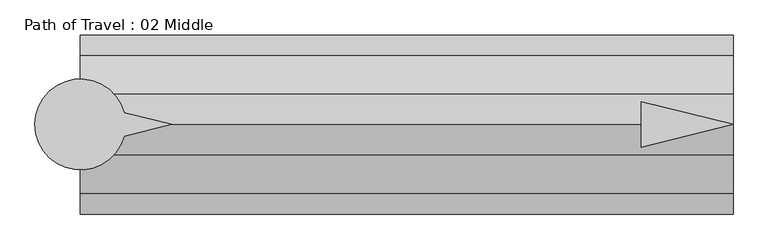
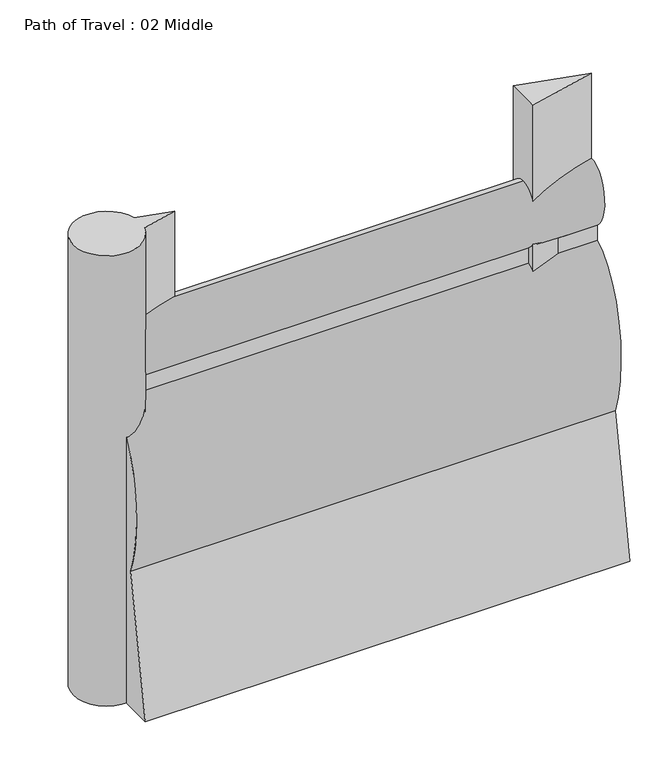
"""IFC4 building model written with IfcOpenShell, lengths in millimetres: proxy geometry, Path of Travel : 02 Middle."""

from ifc_helpers import new_model, si_unit, point, frame, frame_2d, origin, origin_with_axes, place, context, project, spatial, polyline, circle_curve, ellipse_curve, trimmed, segment, composite_curve, outline, extrude, source, transform, mapped, element, save
from ifc_brep_helpers import plane_surface, extruded_surface, advanced_brep


def path_of_travel_02_middle_73e1806b(model_context):
    return source(origin(), model_context, "Body", "SolidModel", [
        advanced_brep(
        [(227.5554837, 0.0, 1727.2), (227.5554837, 42.9018657, 1436.6534209), (227.5554837, 42.9018657, 1363.4763406), (227.5554837, 184.1186263, 643.4144547), (227.5554837, 297.5699544, 0.0), (227.5554837, 145.6574193, 0.0), (227.5554837, 0.0, 584.2), (227.5554837, -145.6574193, 0.0), (227.5554837, -297.5699544, 0.0), (227.5554837, -184.1186263, 643.4144547), (227.5554837, -42.9018657, 1363.4763406), (227.5554837, -42.9018657, 1436.6534209), (2397.3704554, 0.0, 1727.2), (2397.3704554, -42.9018657, 1436.6534209), (2397.3704554, -42.9018657, 1363.4763406), (2397.3704554, -184.1186263, 643.4144547), (2397.3704554, -297.5699544, 0.0), (2397.3704554, -145.6574193, 0.0), (2397.3704554, 0.0, 584.2), (2397.3704554, 145.6574193, 0.0), (2397.3704554, 297.5699544, 0.0), (2397.3704554, 184.1186263, 643.4144547), (2397.3704554, 42.9018657, 1363.4763406), (2397.3704554, 42.9018657, 1436.6534209)],
        [
            (0, 1, ellipse_curve(frame((227.5554837, 0.0, 1574.8), z_axis=(-1.0, 0.0, 0.0), x_axis=(0.0, 0.0, 1.0)), 152.4, 101.6)),
            (1, 2),
            (2, 3, ellipse_curve(frame((227.5554837, 0.0, 914.4), z_axis=(-1.0, 0.0, 0.0), x_axis=(0.0, 0.0, -1.0)), 457.2, 228.6)),
            (3, 4),
            (4, 5),
            (5, 6),
            (6, 7),
            (7, 8),
            (8, 9),
            (9, 10, ellipse_curve(frame((227.5554837, 0.0, 914.4), z_axis=(-1.0, 0.0, 0.0), x_axis=(0.0, 0.0, -1.0)), 457.2, 228.6)),
            (10, 11),
            (11, 0, ellipse_curve(frame((227.5554837, 0.0, 1574.8), z_axis=(-1.0, 0.0, 0.0), x_axis=(0.0, 0.0, 1.0)), 152.4, 101.6)),
            (12, 13, ellipse_curve(frame((2397.3704554, 0.0, 1574.8), z_axis=(1.0, 0.0, 0.0), x_axis=(0.0, 0.0, 1.0)), 152.4, 101.6)),
            (13, 14),
            (14, 15, ellipse_curve(frame((2397.3704554, 0.0, 914.4), z_axis=(1.0, 0.0, 0.0), x_axis=(0.0, 0.0, -1.0)), 457.2, 228.6)),
            (15, 16),
            (16, 17),
            (17, 18),
            (18, 19),
            (19, 20),
            (20, 21),
            (21, 22, ellipse_curve(frame((2397.3704554, 0.0, 914.4), z_axis=(1.0, 0.0, 0.0), x_axis=(0.0, 0.0, -1.0)), 457.2, 228.6)),
            (22, 23),
            (23, 12, ellipse_curve(frame((2397.3704554, 0.0, 1574.8), z_axis=(1.0, 0.0, 0.0), x_axis=(0.0, 0.0, 1.0)), 152.4, 101.6)),
            (0, 12),
            (23, 1),
            (22, 2),
            (21, 3),
            (20, 4),
            (19, 5),
            (18, 6),
            (17, 7),
            (16, 8),
            (15, 9),
            (14, 10),
            (13, 11),
        ],
        [
            plane_surface(frame((227.5554837, 0.0, 0.0), z_axis=(-1.0, 0.0, 0.0), x_axis=(0.0, 0.0, 1.0))),
            plane_surface(frame((2397.3704554, 0.0, 0.0), z_axis=(1.0, 0.0, 0.0), x_axis=(0.0, 0.0, 1.0))),
            extruded_surface(trimmed(ellipse_curve(frame((2397.3704554, 0.0, 1574.8), z_axis=(-1.0, 0.0, 0.0), x_axis=(0.0, 0.0, 1.0)), 152.4, 101.6), [point((2397.3704554, 0.0, 1727.2))], [point((2397.3704554, 42.9018657, 1436.6534209))], True, "CARTESIAN"), (-2169.8149717, 0.0, 0.0), 2169.8149717),
            plane_surface(frame((227.5554837, 42.9018657, 1436.6534209), z_axis=(0.0, 1.0, 0.0), x_axis=(1.0, 0.0, 0.0))),
            extruded_surface(trimmed(ellipse_curve(frame((2397.3704554, 0.0, 914.4), z_axis=(-1.0, 0.0, 0.0), x_axis=(0.0, 0.0, -1.0)), 457.2, 228.6), [point((2397.3704554, 42.9018657, 1363.4763406))], [point((2397.3704554, 184.1186263, 643.4144547))], True, "CARTESIAN"), (-2169.8149717, 0.0, 0.0), 2169.8149717),
            plane_surface(frame((227.5554837, 184.1186263, 643.4144547), z_axis=(0.0, 0.9848077530122078, 0.1736481776669322), x_axis=(1.0, 0.0, 0.0))),
            plane_surface(frame((227.5554837, 297.5699544, 0.0), z_axis=(0.0, 0.0, -1.0), x_axis=(1.0, 0.0, 0.0))),
            plane_surface(frame((227.5554837, 145.6574193, 0.0), z_axis=(0.0, -0.9702957262760199, -0.2419218955995739), x_axis=(1.0, 0.0, 0.0))),
            plane_surface(frame((227.5554837, 0.0, 584.2), z_axis=(0.0, 0.9702957262759961, -0.24192189559966923), x_axis=(1.0, 0.0, 0.0))),
            plane_surface(frame((227.5554837, -145.6574193, 0.0), z_axis=(0.0, 0.0, -1.0), x_axis=(1.0, 0.0, 0.0))),
            plane_surface(frame((227.5554837, -297.5699544, 0.0), z_axis=(0.0, -0.984807753012208, 0.17364817766693066), x_axis=(1.0, 0.0, 0.0))),
            extruded_surface(trimmed(ellipse_curve(frame((2397.3704554, 0.0, 914.4), z_axis=(-1.0, 0.0, 0.0), x_axis=(0.0, 0.0, -1.0)), 457.2, 228.6), [point((2397.3704554, -184.1186263, 643.4144547))], [point((2397.3704554, -42.9018657, 1363.4763406))], True, "CARTESIAN"), (-2169.8149717, 0.0, 0.0), 2169.8149717),
            plane_surface(frame((227.5554837, -42.9018657, 1363.4763406), z_axis=(0.0, -1.0, 0.0), x_axis=(1.0, 0.0, 0.0))),
            extruded_surface(trimmed(ellipse_curve(frame((2397.3704554, 0.0, 1574.8), z_axis=(-1.0, 0.0, 0.0), x_axis=(0.0, 0.0, 1.0)), 152.4, 101.6), [point((2397.3704554, -42.9018657, 1436.6534209))], [point((2397.3704554, 0.0, 1727.2))], True, "CARTESIAN"), (-2169.8149717, 0.0, 0.0), 2169.8149717),
        ],
        [
            (0, [[1, 2, 3, 4, 5, 6, 7, 8, 9, 10, 11, 12]]),
            (1, [[13, 14, 15, 16, 17, 18, 19, 20, 21, 22, 23, 24]]),
            (2, [[-1, 25, -24, 26]]),
            (3, [[-2, -26, -23, 27]]),
            (4, [[-3, -27, -22, 28]]),
            (5, [[-4, -28, -21, 29]]),
            (6, [[-5, -29, -20, 30]]),
            (7, [[-6, -30, -19, 31]]),
            (8, [[-7, -31, -18, 32]]),
            (9, [[-8, -32, -17, 33]]),
            (10, [[-9, -33, -16, 34]]),
            (11, [[-10, -34, -15, 35]]),
            (12, [[-11, -35, -14, 36]]),
            (13, [[-12, -36, -13, -25]]),
        ],
    ),
        extrude(outline(polyline([(2091.3653088, 76.2006338), (2397.3704554, 0.0), (2091.3653088, -76.2006338), (2091.3653088, 76.2006338)])), origin_with_axes(), (0.0, 0.0, 1.0), 2129.5973753),
        extrude(outline(composite_curve([segment(polyline([(372.7837828, 39.4440225), (531.182385, 0.0), (372.7837828, -39.4440225)]), True, "CONTINUOUS"), segment(trimmed(circle_curve(frame_2d((227.2200886, 0.0)), 150.8131956), [point((372.7837828, -39.4440225))], [point((372.7837828, 39.4440225))], False, "CARTESIAN"), True, "CONTINUOUS")], self_intersect=False)), origin_with_axes(), (0.0, 0.0, 1.0), 2129.5973753),
    ])


if __name__ == "__main__":
    model = new_model("IFC4")
    model_context = context("Model", 3, world=origin())
    ifc_project = project(units=[si_unit("LENGTHUNIT", "METRE", prefix="MILLI")], contexts=[model_context])
    site = spatial("IfcSite", under=ifc_project)
    building = spatial("IfcBuilding", under=site)
    placement = place(None, origin())
    path_of_travel_02_middle_shape = path_of_travel_02_middle_73e1806b(model_context)
    element("IfcBuildingElementProxy", 1, Name="Path of Travel : 02 Middle", ObjectType="Path of Travel : 02 Middle", at=placement, inside=building, context=model_context, shape_type="MappedRepresentation", body=[
        mapped(path_of_travel_02_middle_shape, transform((0.0, 0.0, 0.0), x_axis=(1.0, 0.0, 0.0), y_axis=(0.0, 1.0, 0.0), z_axis=(0.0, 0.0, 1.0))),
    ])
    save(model, "model.ifc")

# Revit data of these elements
# Type "Path of Travel : 02 Middle"
#   Path of Egress [instance default] = 4' - 0"
#   built-in parameter 1001306 [instance default] = 4 (stored number, unit not read)
#   Dot at Start = no
#   Arrow in Middle = yes
#   Arrow at End = no
#   Egress Path = none
# Element 1 (IfcBuildingElementProxy, "Path of Travel : 02 Middle")
#   Path of Egress = 7' - 1 109/256"
#   built-in parameter 1001306 = 7.11882 (stored number, unit not read)
#   Materials on its faces: "Egress Path Solid", "solid"
# Materials
#   "Egress Path Solid": class "Unassigned", colour RGB 255 128 64, transparency 0.75, Comments = "Rendering appearance not upgraded "
#   "solid": class "Generic", colour RGB 120 120 120, transparency 0, Cost = 0
